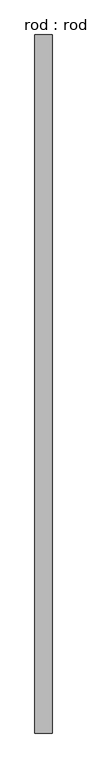
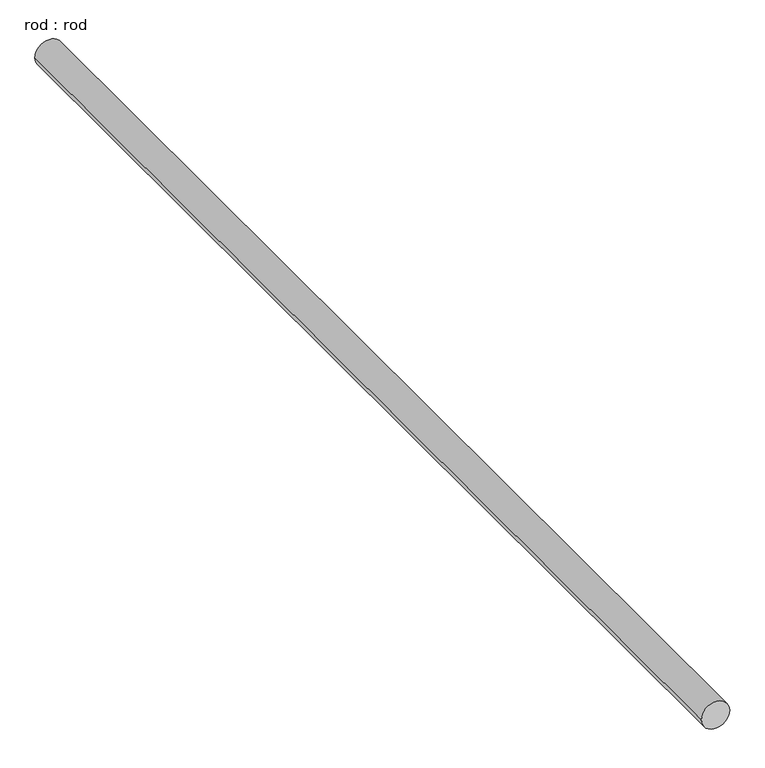
"""IFC4 building model written with IfcOpenShell, lengths in millimetres: proxy geometry, rod : rod."""

from ifc_helpers import new_model, si_unit, point, frame, frame_2d, origin, place, context, project, spatial, circle_curve, trimmed, segment, composite_curve, outline, extrude, source, transform, mapped, element, save


def rod_rod_95942eb3(model_context):
    return source(origin(), model_context, "Body", "SweptSolid", [
        extrude(outline(composite_curve([segment(trimmed(circle_curve(frame_2d((0.0108462, 0.0)), 200.0), [point((0.0108462, 200.0))], [point((0.0108462, -200.0))], False, "CARTESIAN"), True, "CONTINUOUS"), segment(trimmed(circle_curve(frame_2d((0.0108462, 0.0)), 200.0), [point((0.0108462, -200.0))], [point((0.0108462, 200.0))], False, "CARTESIAN"), True, "CONTINUOUS")], self_intersect=False)), frame((0.0, -4063.5213847, 0.0), z_axis=(0.0, 1.0, 0.0), x_axis=(0.0, 0.0, 1.0)), (0.0, 0.0, 1.0), 16312.5),
    ])


if __name__ == "__main__":
    model = new_model("IFC4")
    model_context = context("Model", 3, world=origin())
    ifc_project = project(units=[si_unit("LENGTHUNIT", "METRE", prefix="MILLI")], contexts=[model_context])
    site = spatial("IfcSite", under=ifc_project)
    building = spatial("IfcBuilding", under=site)
    placement = place(None, origin())
    rod_rod_shape = rod_rod_95942eb3(model_context)
    element("IfcBuildingElementProxy", 1, Name="rod : rod", ObjectType="rod : rod", at=placement, inside=building, context=model_context, shape_type="MappedRepresentation", body=[
        mapped(rod_rod_shape, transform((0.0, 0.0, 0.0), x_axis=(1.0, 0.0, 0.0), y_axis=(0.0, 1.0, 0.0), z_axis=(0.0, 0.0, 1.0))),
    ])
    save(model, "model.ifc")

# Revit data of these elements
# Type "rod : rod"
#   Default Elevation = 0
